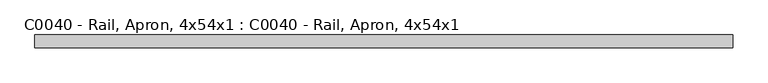
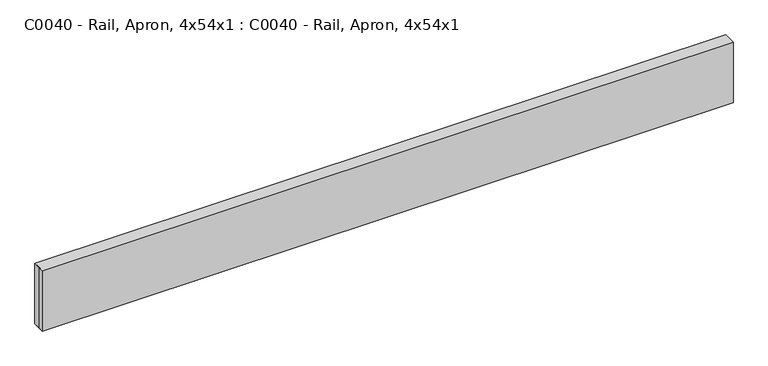
"""IFC4 building model written with IfcOpenShell, lengths in millimetres: proxy geometry, C0040 - Rail, Apron, 4x54x1 : C0040 - Rail, Apron, 4x54x1."""

from ifc_helpers import new_model, si_unit, frame, origin, place, context, project, spatial, polyline, outline, extrude, source, transform, mapped, element, save


def c0040_rail_apron_4x54x1_c0040_rail_apron_4x54x1_1871e43f(model_context):
    return source(origin(), model_context, "Body", "SweptSolid", [
        extrude(outline(polyline([(-685.8, 12.7), (685.8, 12.7), (685.8, -12.7), (-685.8, -12.7), (-685.8, 0.0), (-685.8, 12.7)])), frame((0.0, 0.0, 711.2), z_axis=(0.0, 0.0, 1.0), x_axis=(1.0, 0.0, 0.0)), (0.0, 0.0, 1.0), 127.0),
        extrude(outline(polyline([(685.8, 12.7), (685.8, -12.7), (-685.8, -12.7), (-685.8, 12.7), (685.8, 12.7)])), frame((0.0, 0.0, 711.2), z_axis=(0.0, 0.0, 1.0), x_axis=(1.0, 0.0, 0.0)), (0.0, 0.0, 1.0), 127.0),
    ])


if __name__ == "__main__":
    model = new_model("IFC4")
    model_context = context("Model", 3, world=origin())
    ifc_project = project(units=[si_unit("LENGTHUNIT", "METRE", prefix="MILLI")], contexts=[model_context])
    site = spatial("IfcSite", under=ifc_project)
    building = spatial("IfcBuilding", under=site)
    placement = place(None, origin())
    c0040_rail_apron_4x54x1_c0040_rail_apron_4x54x1_shape = c0040_rail_apron_4x54x1_c0040_rail_apron_4x54x1_1871e43f(model_context)
    element("IfcBuildingElementProxy", 1, Name="C0040 - Rail, Apron, 4x54x1 : C0040 - Rail, Apron, 4x54x1", ObjectType="C0040 - Rail, Apron, 4x54x1 : C0040 - Rail, Apron, 4x54x1", at=placement, inside=building, context=model_context, shape_type="MappedRepresentation", body=[
        mapped(c0040_rail_apron_4x54x1_c0040_rail_apron_4x54x1_shape, transform((0.0, 0.0, 0.0), x_axis=(1.0, 0.0, 0.0), y_axis=(0.0, 1.0, 0.0), z_axis=(0.0, 0.0, 1.0))),
    ])
    save(model, "model.ifc")

# Revit data of these elements
# Project information
#   Room Abbreviation = "TRPE1/TLTU1"
#   Room Description 2-1 = "Treatment, Proctoscopy (LGI) (TRPE1)"
#   Room Description 2-2 = "Toilet (TLTU1)"
#   Sheets - Total = "7"
#   Project Issue Date = "Issue Date"
#   Project Status = "Project Status"
#   Client Name = "Owner"
#   Project Address = "Enter address here"
#   Project Name = "Project Name"
#   Project Number = "Project Number"
#   Publication Date = "1-Feb-16"
# Type "C0040 - Rail, Apron, 4x54x1 : C0040 - Rail, Apron, 4x54x1"
#   Watts2 = "0"
#   Watts1 = "0"
#   Unit_Issue = "EA"
#   UTIL_6_Misc = "-"
#   UTIL_5_NonMedGas = "-"
#   UTIL_4_MiscGas = "-"
#   UTIL_3_MedGas = "-"
#   UTIL_2_Elec = "-"
#   UTIL_1_WaterDrain = "-"
#   Nomenclature = "Rail, Apron, 4x54x1"
#   NSN = "6530"
#   Location [instance default] = ""
#   JSN = "C0040"
#   Fund_Source_VA = "-"
#   Fund_Source_Navy = "-"
#   Fund_Source_Army = "-"
#   Fund_Source_AF = "-"
#   ELEC_Volts2 = "0"
#   ELEC_Volts1 = "0"
#   ELEC_Phase2 = "0"
#   ELEC_Phase1 = "0"
#   ELEC_HertzSwitch = "0"
#   ELEC_HertzDependent = "0"
#   ELEC_Hertz = "0"
#   ELEC_Amps2 = "0"
#   ELEC_Amps1 = "0"
#   DetailDescription = "Apron rail. Also referred to as an apron front, apron panel, or knee space rail. Used to close in front knee space area and/or provide work surface support between two base cabinets or a base cabinet and wall. Apron rails should be ordered in pairs to provide both front and rear work surface support."
#   CAT_VA = "A"
#   CAT_Navy = "A"
#   CAT_IHS = "-"
#   CAT_Army = "A"
#   CAT_AF = "A"
#   BTUperhour = "0"
#   Weight_IP = 16
#   DIM_Width_IP = 4' - 6"
#   DIM_Height_IP = 0' - 5"
#   DIM_Depth_IP = 0' - 1"
# Element 1 (IfcBuildingElementProxy, "C0040 - Rail, Apron, 4x54x1 : C0040 - Rail, Apron, 4x54x1")
#   Location = "TRPE1"
#   Materials on its faces: "EquipSpace"
# Materials
#   "EquipSpace": class "Unassigned", colour RGB 221 217 195, transparency 0.5
